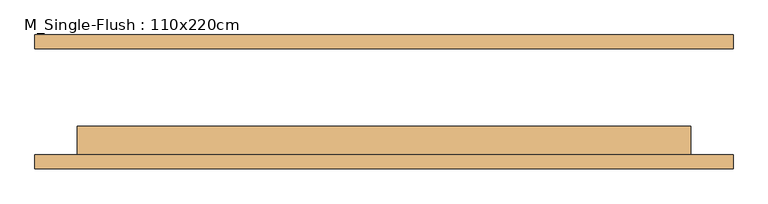
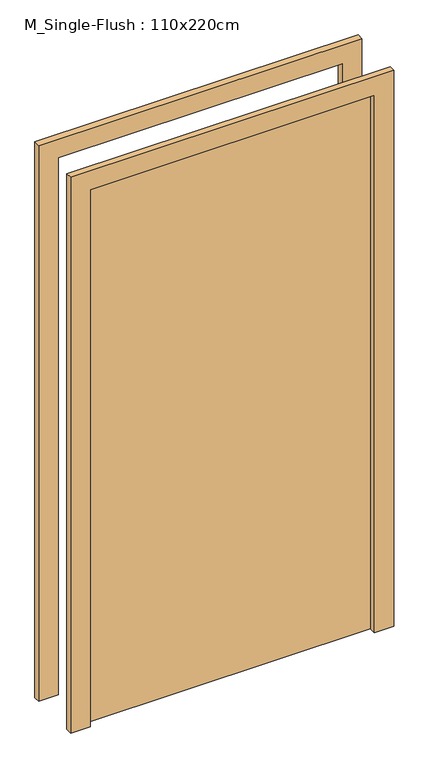
"""IFC4 building model written with IfcOpenShell, lengths in millimetres: door geometry, M_Single-Flush : 110x220cm."""

import ifcopenshell
import ifcopenshell.guid

model = None  # the IFC model being written
_history = None  # IfcOwnerHistory: only IFC2X3 demands one
_inside = {}  # id of a spatial element -> (the spatial element, [elements in it])
_under = {}  # id of a project, library or spatial element -> (it, [spatial elements below it])
_declared = {}  # id of a project -> (the project, [libraries it declares])
_typed = {}  # id of a type object -> (the type object, [elements of that type])
_made_of = {}  # id of a material, layer set ... -> (it, [elements and type objects made of it])


def new_model(schema):
    """Start an empty IFC model of exactly this schema.

    Asked for "IFC4X3", IfcOpenShell would pick the latest addendum, in which some entities
    have other attributes; the version numbers below select the first issue.
    IFC2X3 requires an IfcOwnerHistory on every rooted entity: one is made here for all.
    """
    global model, _history
    if schema == "IFC4X3":
        model = ifcopenshell.file(schema_version=(4, 3, 0, 0))
    else:
        model = ifcopenshell.file(schema=schema)
    _inside.clear()
    _under.clear()
    _declared.clear()
    _typed.clear()
    _made_of.clear()
    _history = None
    if model.schema == "IFC2X3":
        org = make("IfcOrganization", Name="unknown")
        user = make(
            "IfcPersonAndOrganization",
            ThePerson=make("IfcPerson", FamilyName="unknown"),
            TheOrganization=org,
        )
        app = make(
            "IfcApplication",
            ApplicationDeveloper=org,
            Version="unknown",
            ApplicationFullName="unknown",
            ApplicationIdentifier="unknown",
        )
        _history = make(
            "IfcOwnerHistory",
            OwningUser=user,
            OwningApplication=app,
            ChangeAction="ADDED",
            CreationDate=0,
        )
    return model


def make(cls, **values):
    """One entity of the class cls with the attributes given. An attribute that is None is left unset."""
    return model.create_entity(
        cls, **{name: value for name, value in values.items() if value is not None}
    )


def rooted(cls, **values):
    """An entity with a GlobalId (a new one), such as an element, a storey or a relation."""
    return make(cls, GlobalId=ifcopenshell.guid.new(), OwnerHistory=_history, **values)


def si_unit(unit_type, name, prefix=None):
    """IfcSIUnit, for example si_unit("LENGTHUNIT", "METRE", prefix="MILLI")."""
    return make("IfcSIUnit", UnitType=unit_type, Prefix=prefix, Name=name)


def assignment(units):
    """IfcUnitAssignment: the units of a project."""
    return None if units is None else make("IfcUnitAssignment", Units=units)


def point(xyz):
    """IfcCartesianPoint."""
    return None if xyz is None else make("IfcCartesianPoint", Coordinates=xyz)


def direction(xyz):
    """IfcDirection."""
    return None if xyz is None else make("IfcDirection", DirectionRatios=xyz)


def frame(location, z_axis=None, x_axis=None):
    """IfcAxis2Placement3D, a coordinate frame: its origin and axes. An axis left out is left unset."""
    return make(
        "IfcAxis2Placement3D",
        Location=point(location),
        Axis=direction(z_axis),
        RefDirection=direction(x_axis),
    )


def origin():
    """The frame at (0, 0, 0) with its axes left unset."""
    return frame((0.0, 0.0, 0.0))


def origin_with_axes():
    """The frame at (0, 0, 0) with the z axis (0, 0, 1) and the x axis (1, 0, 0) written out."""
    return frame((0.0, 0.0, 0.0), z_axis=(0.0, 0.0, 1.0), x_axis=(1.0, 0.0, 0.0))


def place(relative_to, where):
    """IfcLocalPlacement: puts the frame where relative to a parent placement (None: the world)."""
    return make(
        "IfcLocalPlacement", PlacementRelTo=relative_to, RelativePlacement=where
    )


def context(
    kind, dimensions, precision=None, world=None, true_north=None, identifier=None
):
    """IfcGeometricRepresentationContext, for example the 3D "Model" context."""
    return make(
        "IfcGeometricRepresentationContext",
        ContextIdentifier=identifier,
        ContextType=kind,
        CoordinateSpaceDimension=dimensions,
        Precision=precision,
        WorldCoordinateSystem=world,
        TrueNorth=true_north,
    )


def project(units=None, contexts=None):
    """IfcProject with its units and contexts."""
    return rooted(
        "IfcProject",
        Name="project",
        RepresentationContexts=contexts,
        UnitsInContext=assignment(units),
    )


def spatial(cls, under=None, at=None, **own):
    """A site, building, storey or space (cls), placed at a placement, below another one or the project."""
    s = rooted(cls, ObjectPlacement=at, **own)
    if under is not None:
        _under.setdefault(under.id(), (under, []))[1].append(s)
    return s


def polyline(points):
    """IfcPolyline through the points."""
    return make("IfcPolyline", Points=[point(p) for p in points])


def outline(outer, holes=None, kind="AREA"):
    """IfcArbitraryClosedProfileDef: a profile drawn as a closed curve; with holes, ...WithVoids."""
    if holes is None:
        return make("IfcArbitraryClosedProfileDef", ProfileType=kind, OuterCurve=outer)
    return make(
        "IfcArbitraryProfileDefWithVoids",
        ProfileType=kind,
        OuterCurve=outer,
        InnerCurves=holes,
    )


def extrude(swept, where, along, depth):
    """IfcExtrudedAreaSolid: the profile swept, set in the frame where, extruded along a direction by depth."""
    return make(
        "IfcExtrudedAreaSolid",
        SweptArea=swept,
        Position=where,
        ExtrudedDirection=direction(along),
        Depth=depth,
    )


def shape(context_of_items, identifier, shape_type, items):
    """IfcShapeRepresentation: the items that make up one representation, for example the "Body"."""
    return make(
        "IfcShapeRepresentation",
        ContextOfItems=context_of_items,
        RepresentationIdentifier=identifier,
        RepresentationType=shape_type,
        Items=items,
    )


def source(mapping_origin, context_of_items, identifier, shape_type, items):
    """IfcRepresentationMap: a shape defined once, which mapped items show again and again."""
    return make(
        "IfcRepresentationMap",
        MappingOrigin=mapping_origin,
        MappedRepresentation=shape(context_of_items, identifier, shape_type, items),
    )


def transform(
    local_origin,
    x_axis=None,
    y_axis=None,
    z_axis=None,
    scale=None,
    scale2=None,
    scale3=None,
    uniform=True,
):
    """IfcCartesianTransformationOperator3D, or its non-uniform kind. x_axis, y_axis, z_axis: its Axis1, 2, 3."""
    if uniform:
        return make(
            "IfcCartesianTransformationOperator3D",
            Axis1=direction(x_axis),
            Axis2=direction(y_axis),
            LocalOrigin=point(local_origin),
            Scale=scale,
            Axis3=direction(z_axis),
        )
    return make(
        "IfcCartesianTransformationOperator3DnonUniform",
        Axis1=direction(x_axis),
        Axis2=direction(y_axis),
        LocalOrigin=point(local_origin),
        Scale=scale,
        Axis3=direction(z_axis),
        Scale2=scale2,
        Scale3=scale3,
    )


def mapped(mapping_source, mapping_target):
    """IfcMappedItem: shows the shape of a source again, moved by a transform."""
    return make(
        "IfcMappedItem", MappingSource=mapping_source, MappingTarget=mapping_target
    )


def made_of(thing, what):
    """Note that an element or type object is made of a material, layer set ...; save() writes the relation."""
    if what is not None:
        _made_of.setdefault(what.id(), (what, []))[1].append(thing)
    return thing


def element(
    cls,
    number,
    at=None,
    inside=None,
    cuts=None,
    type_object=None,
    material=None,
    context=None,
    identifier="Body",
    shape_type=None,
    held_by="IfcProductDefinitionShape",
    body=None,
    shapes=None,
    **own,
):
    """One element of the class cls, such as IfcWall. Its Tag is "e" and its number.

    at: its placement. inside: the storey or other place that contains it. cuts: it is an
    opening in that element (IfcRelVoidsElement). A single representation is given by context,
    identifier, shape_type and body (its items); several are given by shapes. held_by: the class
    of the entity that holds the representations. save() writes the other relations.
    """
    e = rooted(cls, Tag="e%d" % number, ObjectPlacement=at, **own)
    if body is not None:
        shapes = [shape(context, identifier, shape_type, body)]
    if shapes is not None:
        e.Representation = make(held_by, Representations=shapes)
    if inside is not None:
        _inside.setdefault(inside.id(), (inside, []))[1].append(e)
    if cuts is not None:
        rooted(
            "IfcRelVoidsElement", RelatingBuildingElement=cuts, RelatedOpeningElement=e
        )
    if type_object is not None:
        _typed.setdefault(type_object.id(), (type_object, []))[1].append(e)
    return made_of(e, material)


def aggregate(whole, parts):
    """IfcRelAggregates: a whole, such as a stair, and the parts it consists of."""
    return rooted("IfcRelAggregates", RelatingObject=whole, RelatedObjects=parts)


def save(model, path):
    """Write the relations noted so far, then the file.

    IfcRelAggregates (storeys below a building ...), IfcRelContainedInSpatialStructure (elements
    in a storey), IfcRelDefinesByType, IfcRelAssociatesMaterial and IfcRelDeclares: one each for
    every whole, place, type object, material and project.
    """
    for whole, parts in _under.values():
        aggregate(whole, parts)
    for where, things in _inside.values():
        rooted(
            "IfcRelContainedInSpatialStructure",
            RelatedElements=things,
            RelatingStructure=where,
        )
    for kind, things in _typed.values():
        rooted("IfcRelDefinesByType", RelatedObjects=things, RelatingType=kind)
    for what, things in _made_of.values():
        rooted("IfcRelAssociatesMaterial", RelatedObjects=things, RelatingMaterial=what)
    for by, libraries in _declared.values():
        rooted("IfcRelDeclares", RelatingContext=by, RelatedDefinitions=libraries)
    model.write(path)


def m_single_flush_110x220cm_75335aee(model_context):
    return source(origin(), model_context, "Body", "SweptSolid", [
        extrude(outline(polyline([(2276.0, -626.0), (0.0, -626.0), (0.0, -550.0), (2200.0, -550.0), (2200.0, 550.0), (0.0, 550.0), (0.0, 626.0), (2276.0, 626.0), (2276.0, -626.0)])), frame((0.0, -120.0, 0.0), z_axis=(0.0, 1.0, 0.0), x_axis=(0.0, 0.0, 1.0)), (0.0, 0.0, 1.0), 25.0),
        extrude(outline(polyline([(2276.0, 626.0), (2276.0, -626.0), (0.0, -626.0), (0.0, -550.0), (2200.0, -550.0), (2200.0, 550.0), (0.0, 550.0), (0.0, 626.0), (2276.0, 626.0)])), frame((0.0, 95.0, 0.0), z_axis=(0.0, 1.0, 0.0), x_axis=(0.0, 0.0, 1.0)), (0.0, 0.0, 1.0), 25.0),
        extrude(outline(polyline([(550.0, -44.0), (550.0, -95.0), (-550.0, -95.0), (-550.0, -44.0), (550.0, -44.0)])), origin_with_axes(), (0.0, 0.0, 1.0), 2200.0),
    ])


if __name__ == "__main__":
    model = new_model("IFC4")
    model_context = context("Model", 3, world=origin())
    ifc_project = project(units=[si_unit("LENGTHUNIT", "METRE", prefix="MILLI")], contexts=[model_context])
    site = spatial("IfcSite", under=ifc_project)
    building = spatial("IfcBuilding", under=site)
    placement = place(None, origin())
    m_single_flush_110x220cm_shape = m_single_flush_110x220cm_75335aee(model_context)
    element("IfcDoor", 1, ObjectType="M_Single-Flush : 110x220cm", at=placement, inside=building, context=model_context, shape_type="MappedRepresentation", body=[
        mapped(m_single_flush_110x220cm_shape, transform((0.0, 0.0, 0.0), x_axis=(1.0, 0.0, 0.0), y_axis=(0.0, 1.0, 0.0), z_axis=(0.0, 0.0, 1.0))),
    ])
    save(model, "model.ifc")

# Revit data of these elements
# Type "M_Single-Flush : 110x220cm"
#   Type Mark = "45"
#   Construction Type Id = "MDOOR"
#   Analytic Construction = "Metal"
#   Thickness = 5.10 cm
#   Heat Transfer Coefficient (U) = 3.7021 W/(m²·K)
#   Height = 220.00 cm
#   Trim Projection Ext = 2.50 cm
#   Trim Projection Int = 2.50 cm
#   Trim Width = 7.60 cm
#   Width = 110.00 cm
#   Define Thermal Properties by = 1
#   Door Material = Door - Panel
#   Frame Material = Door - Frame
#   Visual Light Transmittance = 0
#   Solar Heat Gain Coefficient = 0
#   Function = (empty or 0)
#   Wall Closure = (empty or 0)
# Element 1 (IfcDoor, "M_Single-Flush : 110x220cm")
#   Materials on its faces: "Door - Frame", "Door - Panel"
# Materials
#   "Door - Panel": class "Wood", colour RGB 210 159 95, transparency 0, Cost = 0
#   "Door - Frame": class "Miscellaneous", colour RGB 118 70 51, transparency 0, Cost = 0
